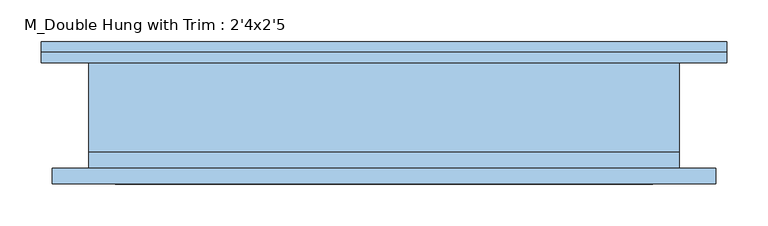
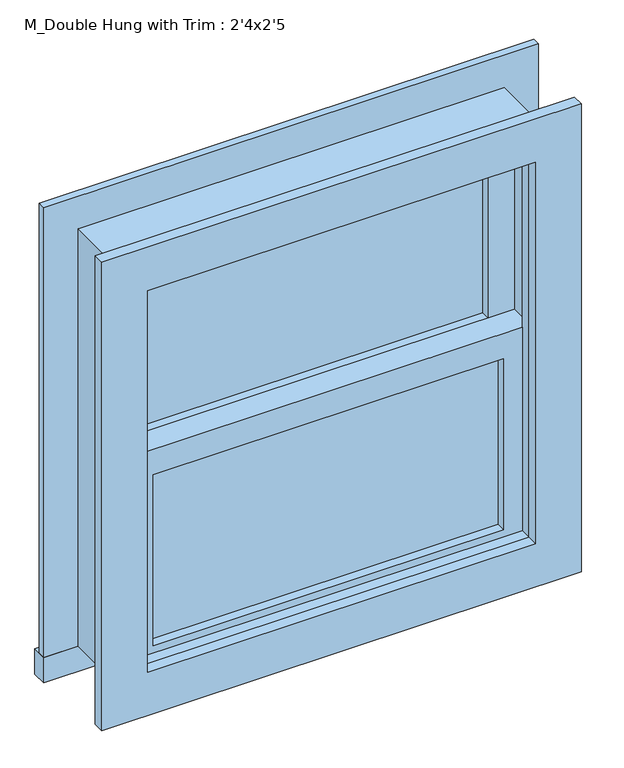
"""IFC4 building model written with IfcOpenShell, lengths in millimetres: window geometry, M_Double Hung with Trim : 2'4x2'5."""

from ifc_helpers import new_model, si_unit, frame, origin, place, context, project, spatial, polyline, outline, extrude, source, transform, mapped, element, save


def m_double_hung_with_trim_2_4x2_5_2372ae1d(model_context):
    return source(origin(), model_context, "Body", "SweptSolid", [
        extrude(outline(polyline([(-292.1, -15.825), (292.1, -15.825), (292.1, -28.525), (-292.1, -28.525), (-292.1, -15.825)])), frame((0.0, 0.0, 628.65), z_axis=(0.0, 0.0, 1.0), x_axis=(1.0, 0.0, 0.0)), (0.0, 0.0, 1.0), 301.625),
        extrude(outline(polyline([(974.725, -336.55), (584.2, -336.55), (584.2, 336.55), (974.725, 336.55), (974.725, -336.55)]), holes=[polyline([(930.275, -292.1), (930.275, 292.1), (628.65, 292.1), (628.65, -292.1), (930.275, -292.1)])]), frame((0.0, -44.4, 0.0), z_axis=(0.0, 1.0, 0.0), x_axis=(0.0, 0.0, 1.0)), (0.0, 0.0, 1.0), 44.45),
        extrude(outline(polyline([(-412.75, 89.2), (412.75, 89.2), (412.75, 63.5), (-412.75, 63.5), (-412.75, 89.2)])), frame((0.0, 0.0, 539.75), z_axis=(0.0, 0.0, 1.0), x_axis=(1.0, 0.0, 0.0)), (0.0, 0.0, 1.0), 44.45),
        extrude(outline(polyline([(1377.95, -412.75), (539.75, -412.75), (539.75, 412.75), (1377.95, 412.75), (1377.95, -412.75)]), holes=[polyline([(1301.75, -336.55), (1301.75, 336.55), (584.2, 336.55), (584.2, -336.55), (1301.75, -336.55)])]), frame((0.0, 63.5, 0.0), z_axis=(0.0, 1.0, 0.0), x_axis=(0.0, 0.0, 1.0)), (0.0, 0.0, 1.0), 13.0),
        extrude(outline(polyline([(1365.25, 400.05), (1365.25, -400.05), (539.75, -400.05), (539.75, 400.05), (1365.25, 400.05)]), holes=[polyline([(1289.05, 323.85), (615.95, 323.85), (615.95, -323.85), (1289.05, -323.85), (1289.05, 323.85)])]), frame((0.0, -82.5, 0.0), z_axis=(0.0, 1.0, 0.0), x_axis=(0.0, 0.0, 1.0)), (0.0, 0.0, 1.0), 19.0),
        extrude(outline(polyline([(292.1, 15.925), (-292.1, 15.925), (-292.1, 28.625), (292.1, 28.625), (292.1, 15.925)])), frame((0.0, 0.0, 974.725), z_axis=(0.0, 0.0, 1.0), x_axis=(1.0, 0.0, 0.0)), (0.0, 0.0, 1.0), 282.575),
        extrude(outline(polyline([(1301.75, -336.55), (930.275, -336.55), (930.275, 336.55), (1301.75, 336.55), (1301.75, -336.55)]), holes=[polyline([(1257.3, -292.1), (1257.3, 292.1), (974.725, 292.1), (974.725, -292.1), (1257.3, -292.1)])]), frame((0.0, 0.05, 0.0), z_axis=(0.0, 1.0, 0.0), x_axis=(0.0, 0.0, 1.0)), (0.0, 0.0, 1.0), 44.45),
        extrude(outline(polyline([(1320.8, -355.6), (584.2, -355.6), (584.2, 355.6), (1320.8, 355.6), (1320.8, -355.6)]), holes=[polyline([(1289.05, -323.85), (1289.05, 323.85), (615.95, 323.85), (615.95, -323.85), (1289.05, -323.85)])]), frame((0.0, -63.5, 0.0), z_axis=(0.0, 1.0, 0.0), x_axis=(0.0, 0.0, 1.0)), (0.0, 0.0, 1.0), 19.1),
        extrude(outline(polyline([(1320.8, 355.6), (1320.8, -355.6), (584.2, -355.6), (584.2, 355.6), (1320.8, 355.6)]), holes=[polyline([(1301.75, 336.55), (603.25, 336.55), (603.25, -336.55), (1301.75, -336.55), (1301.75, 336.55)])]), frame((0.0, -44.4, 0.0), z_axis=(0.0, 1.0, 0.0), x_axis=(0.0, 0.0, 1.0)), (0.0, 0.0, 1.0), 107.9),
    ])


if __name__ == "__main__":
    model = new_model("IFC4")
    model_context = context("Model", 3, world=origin())
    ifc_project = project(units=[si_unit("LENGTHUNIT", "METRE", prefix="MILLI")], contexts=[model_context])
    site = spatial("IfcSite", under=ifc_project)
    building = spatial("IfcBuilding", under=site)
    placement = place(None, origin())
    m_double_hung_with_trim_2_4x2_5_shape = m_double_hung_with_trim_2_4x2_5_2372ae1d(model_context)
    element("IfcWindow", 1, ObjectType="M_Double Hung with Trim : 2'4x2'5", at=placement, inside=building, context=model_context, shape_type="MappedRepresentation", body=[
        mapped(m_double_hung_with_trim_2_4x2_5_shape, transform((0.0, 0.0, 0.0), x_axis=(1.0, 0.0, 0.0), y_axis=(0.0, 1.0, 0.0), z_axis=(0.0, 0.0, 1.0))),
    ])
    save(model, "model.ifc")

# Revit data of these elements
# Type "M_Double Hung with Trim : 2'4x2'5"
#   Type Mark = "69"
#   Construction Type Id = "GSP4R"
#   Analytic Construction = "1/8 in Pilkington single glazing"
#   Visual Light Transmittance = 0.9
#   Thermal Resistance (R) = 0.271106 (m²·K)/W
#   Solar Heat Gain Coefficient = 0.78
#   Heat Transfer Coefficient (U) = 3.6886 W/(m²·K)
#   Height = 2' - 5"
#   Default Sill Height = 1' - 11"
#   Trim Projection - Ext. = 0' - 0.51181"
#   Trim Projection - Int. = 0' - 0.74803"
#   Trim Width - Exterior = 0' - 3"
#   Trim Width - Interior = 0' - 3"
#   Width = 2' - 4"
#   Window Inset = 0' - 0.74803"
#   Glass Pane Material = EXISTING WINDOW
#   Sash = Trim
#   Trim Exterior Material = Trim
#   Trim Interior Material = Trim
#   Wall Closure = (empty or 0)
# Element 1 (IfcWindow, "M_Double Hung with Trim : 2'4x2'5")
#   Materials on its faces: "Trim", "EXISTING WINDOW"
# Materials
#   "EXISTING WINDOW": class "Glass", colour RGB 218 227 224, transparency 0.85, Description = "Soda Lime Glass", Cost = 0
#   "Trim": class "Wood", colour RGB 250 251 245, transparency 0, Cost = 0
